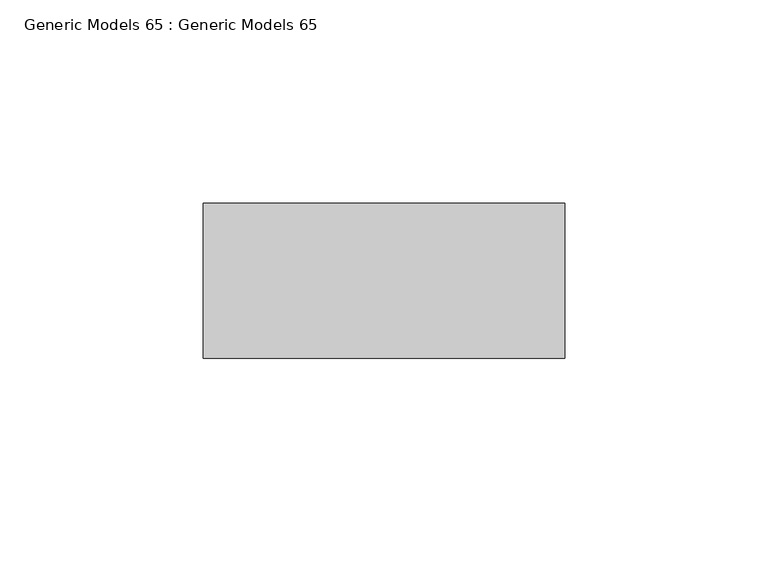
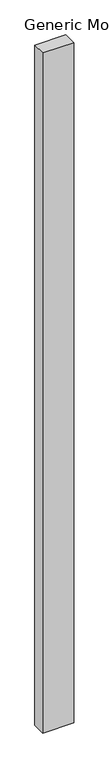
"""IFC4 building model written with IfcOpenShell, lengths in millimetres: proxy geometry, Generic Models 65 : Generic Models 65."""

import ifcopenshell
import ifcopenshell.guid

model = None  # the IFC model being written
_history = None  # IfcOwnerHistory: only IFC2X3 demands one
_inside = {}  # id of a spatial element -> (the spatial element, [elements in it])
_under = {}  # id of a project, library or spatial element -> (it, [spatial elements below it])
_declared = {}  # id of a project -> (the project, [libraries it declares])
_typed = {}  # id of a type object -> (the type object, [elements of that type])
_made_of = {}  # id of a material, layer set ... -> (it, [elements and type objects made of it])


def new_model(schema):
    """Start an empty IFC model of exactly this schema.

    Asked for "IFC4X3", IfcOpenShell would pick the latest addendum, in which some entities
    have other attributes; the version numbers below select the first issue.
    IFC2X3 requires an IfcOwnerHistory on every rooted entity: one is made here for all.
    """
    global model, _history
    if schema == "IFC4X3":
        model = ifcopenshell.file(schema_version=(4, 3, 0, 0))
    else:
        model = ifcopenshell.file(schema=schema)
    _inside.clear()
    _under.clear()
    _declared.clear()
    _typed.clear()
    _made_of.clear()
    _history = None
    if model.schema == "IFC2X3":
        org = make("IfcOrganization", Name="unknown")
        user = make(
            "IfcPersonAndOrganization",
            ThePerson=make("IfcPerson", FamilyName="unknown"),
            TheOrganization=org,
        )
        app = make(
            "IfcApplication",
            ApplicationDeveloper=org,
            Version="unknown",
            ApplicationFullName="unknown",
            ApplicationIdentifier="unknown",
        )
        _history = make(
            "IfcOwnerHistory",
            OwningUser=user,
            OwningApplication=app,
            ChangeAction="ADDED",
            CreationDate=0,
        )
    return model


def make(cls, **values):
    """One entity of the class cls with the attributes given. An attribute that is None is left unset."""
    return model.create_entity(
        cls, **{name: value for name, value in values.items() if value is not None}
    )


def rooted(cls, **values):
    """An entity with a GlobalId (a new one), such as an element, a storey or a relation."""
    return make(cls, GlobalId=ifcopenshell.guid.new(), OwnerHistory=_history, **values)


def si_unit(unit_type, name, prefix=None):
    """IfcSIUnit, for example si_unit("LENGTHUNIT", "METRE", prefix="MILLI")."""
    return make("IfcSIUnit", UnitType=unit_type, Prefix=prefix, Name=name)


def assignment(units):
    """IfcUnitAssignment: the units of a project."""
    return None if units is None else make("IfcUnitAssignment", Units=units)


def point(xyz):
    """IfcCartesianPoint."""
    return None if xyz is None else make("IfcCartesianPoint", Coordinates=xyz)


def direction(xyz):
    """IfcDirection."""
    return None if xyz is None else make("IfcDirection", DirectionRatios=xyz)


def frame(location, z_axis=None, x_axis=None):
    """IfcAxis2Placement3D, a coordinate frame: its origin and axes. An axis left out is left unset."""
    return make(
        "IfcAxis2Placement3D",
        Location=point(location),
        Axis=direction(z_axis),
        RefDirection=direction(x_axis),
    )


def origin():
    """The frame at (0, 0, 0) with its axes left unset."""
    return frame((0.0, 0.0, 0.0))


def place(relative_to, where):
    """IfcLocalPlacement: puts the frame where relative to a parent placement (None: the world)."""
    return make(
        "IfcLocalPlacement", PlacementRelTo=relative_to, RelativePlacement=where
    )


def context(
    kind, dimensions, precision=None, world=None, true_north=None, identifier=None
):
    """IfcGeometricRepresentationContext, for example the 3D "Model" context."""
    return make(
        "IfcGeometricRepresentationContext",
        ContextIdentifier=identifier,
        ContextType=kind,
        CoordinateSpaceDimension=dimensions,
        Precision=precision,
        WorldCoordinateSystem=world,
        TrueNorth=true_north,
    )


def project(units=None, contexts=None):
    """IfcProject with its units and contexts."""
    return rooted(
        "IfcProject",
        Name="project",
        RepresentationContexts=contexts,
        UnitsInContext=assignment(units),
    )


def spatial(cls, under=None, at=None, **own):
    """A site, building, storey or space (cls), placed at a placement, below another one or the project."""
    s = rooted(cls, ObjectPlacement=at, **own)
    if under is not None:
        _under.setdefault(under.id(), (under, []))[1].append(s)
    return s


def polyline(points):
    """IfcPolyline through the points."""
    return make("IfcPolyline", Points=[point(p) for p in points])


def outline(outer, holes=None, kind="AREA"):
    """IfcArbitraryClosedProfileDef: a profile drawn as a closed curve; with holes, ...WithVoids."""
    if holes is None:
        return make("IfcArbitraryClosedProfileDef", ProfileType=kind, OuterCurve=outer)
    return make(
        "IfcArbitraryProfileDefWithVoids",
        ProfileType=kind,
        OuterCurve=outer,
        InnerCurves=holes,
    )


def extrude(swept, where, along, depth):
    """IfcExtrudedAreaSolid: the profile swept, set in the frame where, extruded along a direction by depth."""
    return make(
        "IfcExtrudedAreaSolid",
        SweptArea=swept,
        Position=where,
        ExtrudedDirection=direction(along),
        Depth=depth,
    )


def shape(context_of_items, identifier, shape_type, items):
    """IfcShapeRepresentation: the items that make up one representation, for example the "Body"."""
    return make(
        "IfcShapeRepresentation",
        ContextOfItems=context_of_items,
        RepresentationIdentifier=identifier,
        RepresentationType=shape_type,
        Items=items,
    )


def source(mapping_origin, context_of_items, identifier, shape_type, items):
    """IfcRepresentationMap: a shape defined once, which mapped items show again and again."""
    return make(
        "IfcRepresentationMap",
        MappingOrigin=mapping_origin,
        MappedRepresentation=shape(context_of_items, identifier, shape_type, items),
    )


def transform(
    local_origin,
    x_axis=None,
    y_axis=None,
    z_axis=None,
    scale=None,
    scale2=None,
    scale3=None,
    uniform=True,
):
    """IfcCartesianTransformationOperator3D, or its non-uniform kind. x_axis, y_axis, z_axis: its Axis1, 2, 3."""
    if uniform:
        return make(
            "IfcCartesianTransformationOperator3D",
            Axis1=direction(x_axis),
            Axis2=direction(y_axis),
            LocalOrigin=point(local_origin),
            Scale=scale,
            Axis3=direction(z_axis),
        )
    return make(
        "IfcCartesianTransformationOperator3DnonUniform",
        Axis1=direction(x_axis),
        Axis2=direction(y_axis),
        LocalOrigin=point(local_origin),
        Scale=scale,
        Axis3=direction(z_axis),
        Scale2=scale2,
        Scale3=scale3,
    )


def mapped(mapping_source, mapping_target):
    """IfcMappedItem: shows the shape of a source again, moved by a transform."""
    return make(
        "IfcMappedItem", MappingSource=mapping_source, MappingTarget=mapping_target
    )


def made_of(thing, what):
    """Note that an element or type object is made of a material, layer set ...; save() writes the relation."""
    if what is not None:
        _made_of.setdefault(what.id(), (what, []))[1].append(thing)
    return thing


def element(
    cls,
    number,
    at=None,
    inside=None,
    cuts=None,
    type_object=None,
    material=None,
    context=None,
    identifier="Body",
    shape_type=None,
    held_by="IfcProductDefinitionShape",
    body=None,
    shapes=None,
    **own,
):
    """One element of the class cls, such as IfcWall. Its Tag is "e" and its number.

    at: its placement. inside: the storey or other place that contains it. cuts: it is an
    opening in that element (IfcRelVoidsElement). A single representation is given by context,
    identifier, shape_type and body (its items); several are given by shapes. held_by: the class
    of the entity that holds the representations. save() writes the other relations.
    """
    e = rooted(cls, Tag="e%d" % number, ObjectPlacement=at, **own)
    if body is not None:
        shapes = [shape(context, identifier, shape_type, body)]
    if shapes is not None:
        e.Representation = make(held_by, Representations=shapes)
    if inside is not None:
        _inside.setdefault(inside.id(), (inside, []))[1].append(e)
    if cuts is not None:
        rooted(
            "IfcRelVoidsElement", RelatingBuildingElement=cuts, RelatedOpeningElement=e
        )
    if type_object is not None:
        _typed.setdefault(type_object.id(), (type_object, []))[1].append(e)
    return made_of(e, material)


def aggregate(whole, parts):
    """IfcRelAggregates: a whole, such as a stair, and the parts it consists of."""
    return rooted("IfcRelAggregates", RelatingObject=whole, RelatedObjects=parts)


def save(model, path):
    """Write the relations noted so far, then the file.

    IfcRelAggregates (storeys below a building ...), IfcRelContainedInSpatialStructure (elements
    in a storey), IfcRelDefinesByType, IfcRelAssociatesMaterial and IfcRelDeclares: one each for
    every whole, place, type object, material and project.
    """
    for whole, parts in _under.values():
        aggregate(whole, parts)
    for where, things in _inside.values():
        rooted(
            "IfcRelContainedInSpatialStructure",
            RelatedElements=things,
            RelatingStructure=where,
        )
    for kind, things in _typed.values():
        rooted("IfcRelDefinesByType", RelatedObjects=things, RelatingType=kind)
    for what, things in _made_of.values():
        rooted("IfcRelAssociatesMaterial", RelatedObjects=things, RelatingMaterial=what)
    for by, libraries in _declared.values():
        rooted("IfcRelDeclares", RelatingContext=by, RelatedDefinitions=libraries)
    model.write(path)


def generic_models_65_generic_models_65_eaa428f0(model_context):
    return source(origin(), model_context, "Body", "SweptSolid", [
        extrude(outline(polyline([(51003.2, 592.1375), (50914.3, 592.1375), (50914.3, 630.2375), (51003.2, 630.2375), (51003.2, 592.1375)])), frame((0.0, 0.0, 3086.1), z_axis=(0.0, 0.0, 1.0), x_axis=(1.0, 0.0, 0.0)), (0.0, 0.0, 1.0), 2060.178125),
    ])


if __name__ == "__main__":
    model = new_model("IFC4")
    model_context = context("Model", 3, world=origin())
    ifc_project = project(units=[si_unit("LENGTHUNIT", "METRE", prefix="MILLI")], contexts=[model_context])
    site = spatial("IfcSite", under=ifc_project)
    building = spatial("IfcBuilding", under=site)
    placement = place(None, origin())
    generic_models_65_generic_models_65_shape = generic_models_65_generic_models_65_eaa428f0(model_context)
    element("IfcBuildingElementProxy", 1, Name="Generic Models 65 : Generic Models 65", ObjectType="Generic Models 65 : Generic Models 65", at=placement, inside=building, context=model_context, shape_type="MappedRepresentation", body=[
        mapped(generic_models_65_generic_models_65_shape, transform((0.0, 0.0, 0.0), x_axis=(1.0, 0.0, 0.0), y_axis=(0.0, 1.0, 0.0), z_axis=(0.0, 0.0, 1.0))),
    ])
    save(model, "model.ifc")

# Revit data of these elements
# Element 1 (IfcBuildingElementProxy, "Generic Models 65 : Generic Models 65")
#   Materials on its faces: "2X WOOD STUD - SEE 'WALL TAG' & 'LAYER MATERIAL SCHEDULE' FOR SPACING & INSULATION TREATMENT, IF APPLICAPLE"
# Materials
#   "2X WOOD STUD - SEE 'WALL TAG' & 'LAYER MATERIAL SCHEDULE' FOR SPACING & INSULATION TREATMENT, IF APPLICAPLE": class "Wood", colour RGB 234 198 147, transparency 0, Description = "Pinus Echinata", Cost = 0
